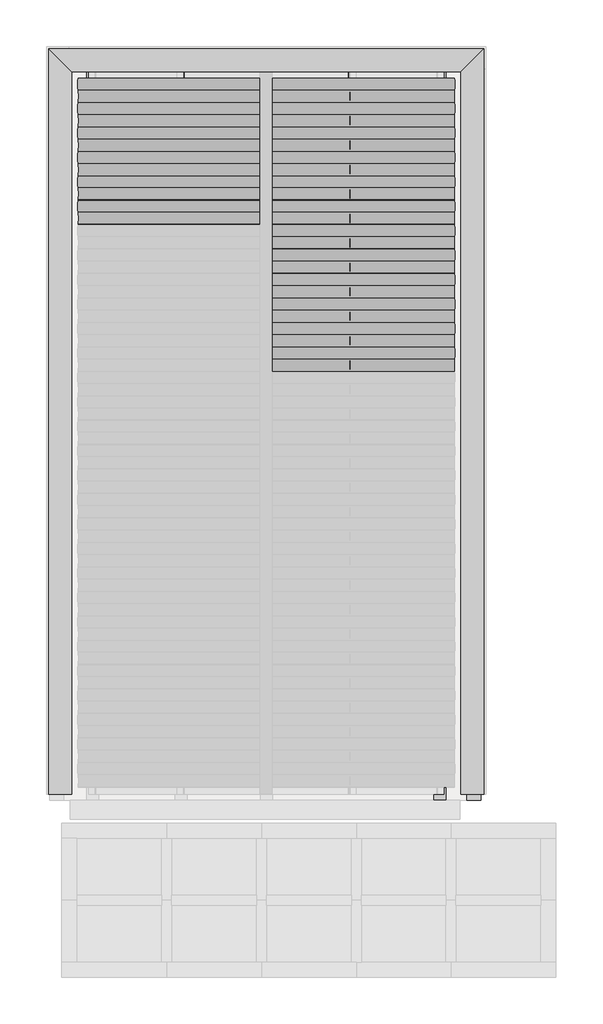
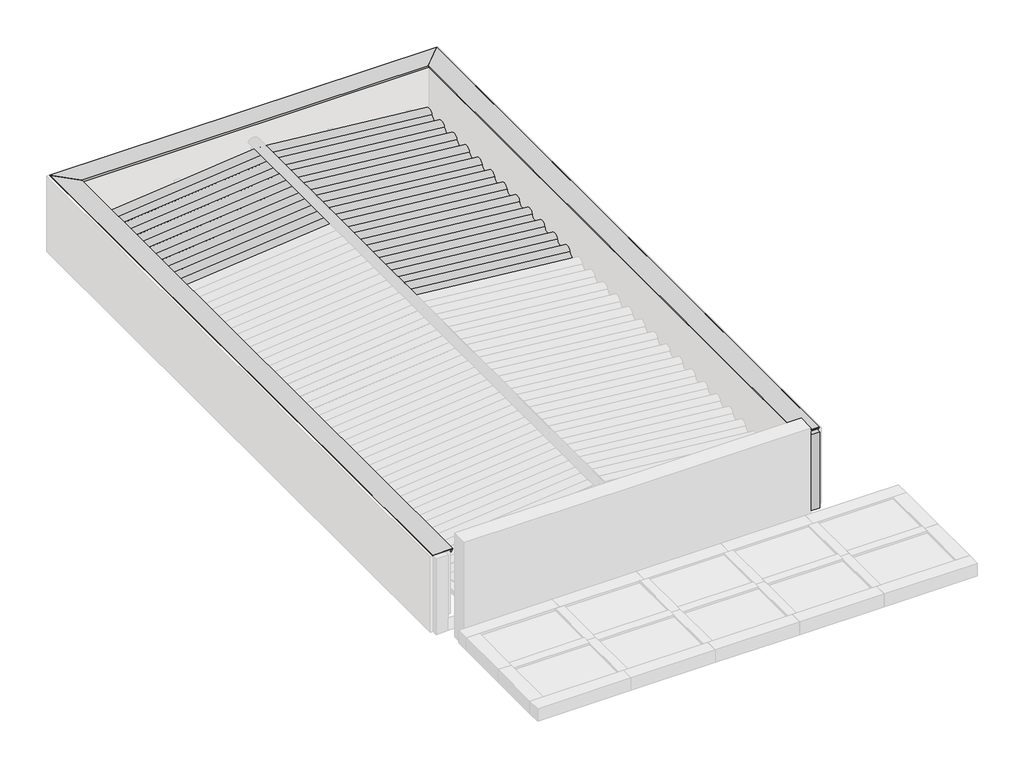
# One storey, part 3 of 3: 32 beams, 11 columns, 2 proxies.
# Revit data of these elements (continued)
# Elements 2, 4, 8, 9, 11, 12 (IfcBeam, "Madeira de lei : Berço 6x12cm") (continued)
#   Comments = ""
#   Uso = "TELHADOS ESTRUTURAS"
#   Compr Cmcl = 7.00 m
#   Structural Material = .MADEIRAMENTO
#   Phase Created = CC_AP
#   Materials on its faces: ".MADEIRAMENTO"
# Element 13 (IfcBeam, "TQS - Viga retangular : 14.0 x 90.0")
#   Uso = "ESTRUTURA"
#   Titulo = "V101"
#   Chave = "-1268"
#   Tipo Elemento = "Viga"
#   SHA1 = "A1785ED040BEC30A264D2E01D04E188751E22668"
#   Revisão = ""
#   Tipo de carga = ""
#   Divisor de flexao = ""
#   Secao = ""
#   Configuracao = ""
#   Angulo (graus) = ""
#   Detalhamento = ""
#   Casos de vento manual = ""
#   Tipo = ""
#   Alcas = ""
#   Furos = ""
#   Pino = ""
#   Distribuicao = ""
#   Solidarizado = ""
#   Solidarizar na montagem = ""
#   Unir com o próximo = ""
#   Grupo pre moldado = ""
#   Verificado = ""
#   Concreto C = ""
#   Taxa de armadura (kgf/m³) = 0
#   Carga (tf/m²) = 0
#   Carga (tf/m) = 0
#   Carga (tf) = 0
#   Altura = 0.90 m
#   Rebaixo = -0.75 m
#   Largura = 0.14 m
#   Distancia a face = 0.00 m
#   Distancia ao eixo = 0.00 m
#   Altura gerber esquerda = 0.00 m
#   Largura gerber esquerda = 0.00 m
#   Altura gerber direita = 0.00 m
#   Largura gerber direita = 0.00 m
#   Resultado de Ensaios fck (MPa) = 0
#   Unique TQS ID = -1268
#   Principal = yes
#   Structural Material = none
#   Phase Created = CC_PE
# Element 14 (IfcBeam, "TQS - Viga retangular : 14.0 x 90.0")
#   Uso = "ESTRUTURA"
#   Titulo = "V104"
#   Chave = "-1270"
#   Tipo Elemento = "Viga"
#   SHA1 = "0A21AF0D9A5F34D6093C65F9A93BBB9D744C094D"
#   Revisão = ""
#   Tipo de carga = ""
#   Divisor de flexao = ""
#   Secao = ""
#   Configuracao = ""
#   Angulo (graus) = ""
#   Detalhamento = ""
#   Casos de vento manual = ""
#   Tipo = ""
#   Alcas = ""
#   Furos = ""
#   Pino = ""
#   Distribuicao = ""
#   Solidarizado = ""
#   Solidarizar na montagem = ""
#   Unir com o próximo = ""
#   Grupo pre moldado = ""
#   Verificado = ""
#   Concreto C = ""
#   Taxa de armadura (kgf/m³) = 0
#   Carga (tf/m²) = 0
#   Carga (tf/m) = 0
#   Carga (tf) = 0
#   Altura = 0.90 m
#   Rebaixo = -0.75 m
#   Largura = 0.14 m
#   Distancia a face = 0.00 m
#   Distancia ao eixo = 0.00 m
#   Altura gerber esquerda = 0.00 m
#   Largura gerber esquerda = 0.00 m
#   Altura gerber direita = 0.00 m
#   Largura gerber direita = 0.00 m
#   Resultado de Ensaios fck (MPa) = 0
#   Unique TQS ID = -1270
#   Principal = yes
#   Structural Material = none
#   Phase Created = CC_PE
# Elements 15, 16, 17, 18, 19, 20, 21, 22, 23, 24, 25, 26, 27, 28, 29, 30, 31, 32 (IfcBeam, "Telha Ondulada : Fibrocimento")
#   Uso = "TELHADOS TELHAS"
#   Phase Created = CC_AP
#   Materials on its faces: ".TELHA DE FIBROCIMENTO"
# Elements 33, 34 (IfcBuildingElementProxy, ".CC_RUFO_PINGADEIRA_22 cm")
#   Uso = "RUFOS COB. GARAGEM"
#   Phase Created = CC_PE
#   Materials on its faces: ".ALUMÍNIO COM PINTURA LÁTEX BRANCA"
# Elements 35, 36, 37, 38, 39, 40, 41, 42, 43, 44, 45 (IfcColumn, "Madeira de lei-Coluna : Pontalete 6X16cm")
#   Comments = ""
#   Uso = "TELHADOS ESTRUTURAS"
#   Compr Cmcl = 2.00 m
#   Structural Material = .MADEIRAMENTO
#   Phase Created = CC_AP
#   Materials on its faces: ".MADEIRAMENTO"
# Materials
#   ".TELHA DE FIBROCIMENTO": class "CC_TELHADO", colour RGB 77 77 76, transparency 0, Description = "TELHA ONDULADA FIBROCIMENTO", Cost = 0
#   ".MADEIRAMENTO": class ".CC_MADEIRAS", colour RGB 212 179 113, transparency 0, Cost = 0
#   ".ALUMÍNIO COM PINTURA LÁTEX BRANCA": class "Generic", colour RGB 250 250 250, transparency 0, Cost = 0
